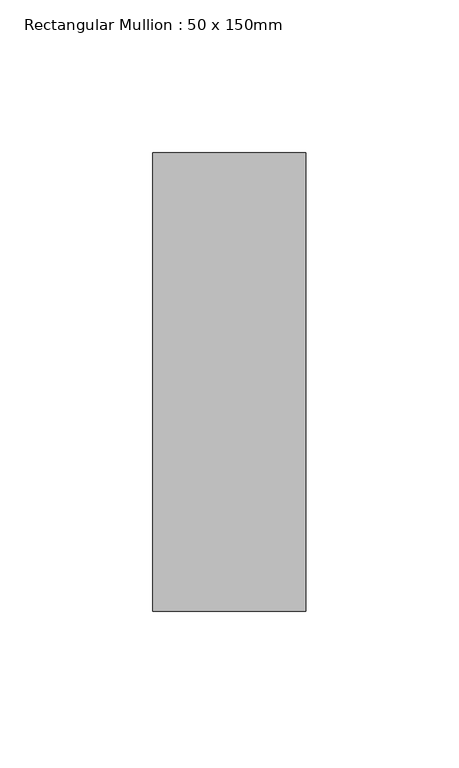
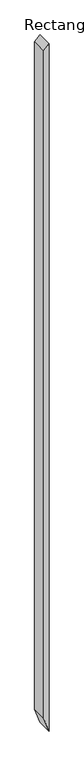
"""IFC4 building model written with IfcOpenShell, lengths in millimetres: member geometry, Rectangular Mullion : 50 x 150mm."""

from ifc_helpers import new_model, si_unit, frame, origin, place, context, project, spatial, polyline, outline, extrude, source, transform, mapped, element, save


def rectangular_mullion_50_x_150mm_835307d9(model_context):
    return source(origin(), model_context, "Body", "SweptSolid", [
        extrude(outline(polyline([(0.0, 0.0), (-53.1084457, -50.0), (-6798.2667293, -50.0), (-6948.5596255, 0.0), (0.0, 0.0)])), frame((0.0, -75.0, 0.0), z_axis=(0.0, 1.0, 0.0), x_axis=(0.0, 0.0, 1.0)), (0.0, 0.0, 1.0), 150.0),
    ])


if __name__ == "__main__":
    model = new_model("IFC4")
    model_context = context("Model", 3, world=origin())
    ifc_project = project(units=[si_unit("LENGTHUNIT", "METRE", prefix="MILLI")], contexts=[model_context])
    site = spatial("IfcSite", under=ifc_project)
    building = spatial("IfcBuilding", under=site)
    placement = place(None, origin())
    rectangular_mullion_50_x_150mm_shape = rectangular_mullion_50_x_150mm_835307d9(model_context)
    element("IfcMember", 1, ObjectType="Rectangular Mullion : 50 x 150mm", at=placement, inside=building, context=model_context, shape_type="MappedRepresentation", body=[
        mapped(rectangular_mullion_50_x_150mm_shape, transform((0.0, 0.0, 0.0), x_axis=(1.0, 0.0, 0.0), y_axis=(0.0, 1.0, 0.0), z_axis=(0.0, 0.0, 1.0))),
    ])
    save(model, "model.ifc")

# Revit data of these elements
# Type "Rectangular Mullion : 50 x 150mm"
#   built-in parameter 1007304 = 0.492126 (stored number, unit not read)
#   built-in parameter 1007301 = 0.082021 (stored number, unit not read)
#   built-in parameter 1007300 = 0.082021 (stored number, unit not read)
# Element 1 (IfcMember, "Rectangular Mullion : 50 x 150mm")
#   Materials on its faces: "Metal - Aluminium"
# Materials
#   "Metal - Aluminium": class "Metal", colour RGB 247 247 247, transparency 0
